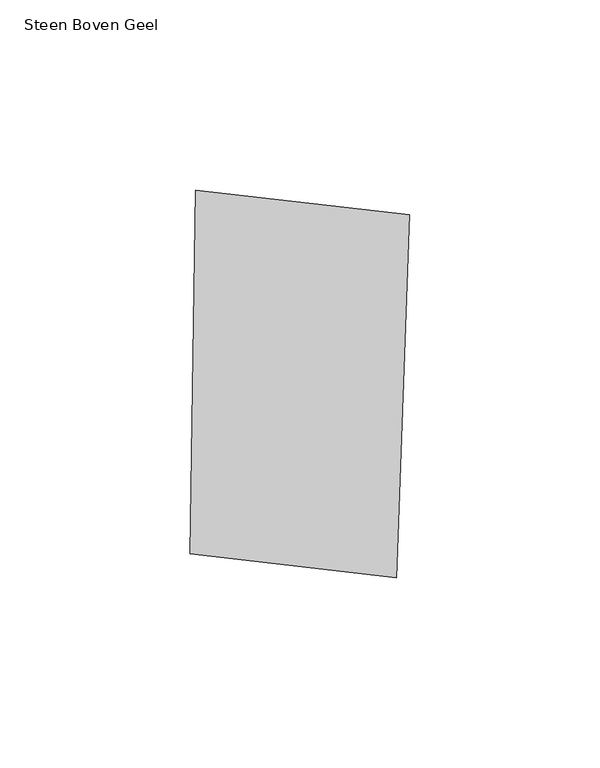
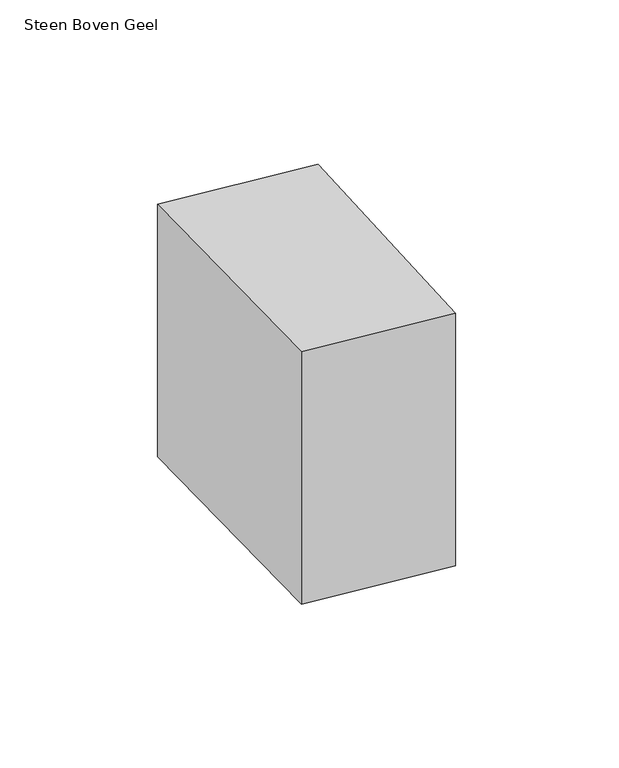
"""IFC4 building model written with IfcOpenShell, lengths in millimetres: proxy geometry, 00_GMA_steen_versie_4 : Steen Boven Geel."""

from ifc_helpers import new_model, si_unit, origin, origin_with_axes, place, context, project, spatial, polyline, outline, extrude, source, transform, mapped, element, save


def steen_boven_geel_ce53416e(model_context):
    return source(origin(), model_context, "Body", "SweptSolid", [
        extrude(outline(polyline([(102.4056604, 119.2826454), (98.9467996, 24.0426664), (44.7452443, 30.2359811), (46.1063142, 125.7242855), (102.4056604, 119.2826454)])), origin_with_axes(), (0.0, 0.0, 1.0), 100.0),
    ])


if __name__ == "__main__":
    model = new_model("IFC4")
    model_context = context("Model", 3, world=origin())
    ifc_project = project(units=[si_unit("LENGTHUNIT", "METRE", prefix="MILLI")], contexts=[model_context])
    site = spatial("IfcSite", under=ifc_project)
    building = spatial("IfcBuilding", under=site)
    placement = place(None, origin())
    steen_boven_geel_shape = steen_boven_geel_ce53416e(model_context)
    element("IfcBuildingElementProxy", 1, Name="00_GMA_steen_versie_4 : Steen Boven Geel", ObjectType="00_GMA_steen_versie_4 : Steen Boven Geel", at=placement, inside=building, context=model_context, shape_type="MappedRepresentation", body=[
        mapped(steen_boven_geel_shape, transform((0.0, 0.0, 0.0), x_axis=(1.0, 0.0, 0.0), y_axis=(0.0, 1.0, 0.0), z_axis=(0.0, 0.0, 1.0))),
    ])
    save(model, "model.ifc")

# Revit data of these elements
# Type "00_GMA_steen_versie_4 : Steen Boven Geel"
#   StootVoegHalfBoven [instance default] = 5 mm
#   StootVoegHalf [instance default] = 5 mm
#   StootVoegBreedteOnder = 10 mm
#   StootVoegBreedteBoven = 10 mm
#   Steendikte = 100 mm
#   LintVoegOnderHalf = 5 mm
#   LintVoegOnder = 10 mm
#   LintVoegBovenHalf = 0 mm
#   LintVoegBoven = 0 mm
#   materiaal = 21_steen_geel
#   MateriaalVoeg = none
#   Default Elevation = 0
# Element 1 (IfcBuildingElementProxy, "00_GMA_steen_versie_4 : Steen Boven Geel")
#   Materials on its faces: "21_steen_geel"
# Materials
#   "21_steen_geel": class "Unassigned", colour RGB 202 202 0, transparency 0, Cost = 0
